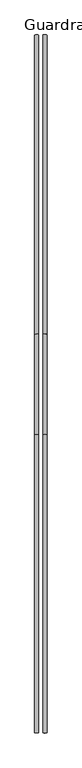
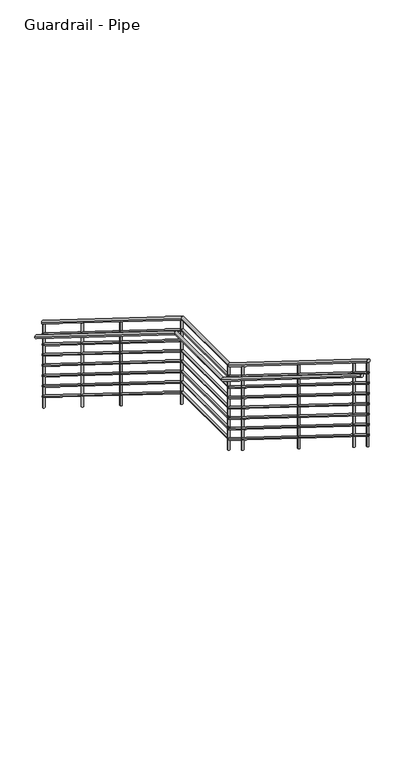
"""IFC4 building model written with IfcOpenShell, lengths in millimetres: railing geometry, Guardrail - Pipe."""

from ifc_helpers import new_model, si_unit, point, frame, frame_2d, origin, place, context, project, spatial, circle_curve, ellipse_curve, trimmed, segment, composite_curve, outline, extrude, source, transform, mapped, element, save
from ifc_brep_helpers import plane_surface, cylinder_surface, advanced_brep


def guardrail_pipe_c5471f49(model_context):
    return source(origin(), model_context, "Body", "SolidModel", [
        advanced_brep(
        [(-2187.3939612, 2884.909643, -2439.0768639), (-2225.4939612, 2884.909643, -2439.0768639), (-2187.3939612, 85.4582154, -693.9642857), (-2225.4939612, 85.4582154, -693.9642857), (-2187.3939612, -854.3417846, -693.9642857), (-2225.4939612, -854.3417846, -693.9642857), (-2187.3939612, -3642.890357, 1044.3517075), (-2225.4939612, -3642.890357, 1044.3517075)],
        [
            (0, 1, ellipse_curve(frame((-2206.4439612, 2884.909643, -2439.0768639), z_axis=(0.0, 1.0, 0.0), x_axis=(0.0, 0.0, -1.0)), 22.4482925, 19.05)),
            (1, 0, ellipse_curve(frame((-2206.4439612, 2884.909643, -2439.0768639), z_axis=(0.0, 1.0, 0.0), x_axis=(0.0, 0.0, -1.0)), 22.4482925, 19.05)),
            (0, 2),
            (2, 3, ellipse_curve(frame((-2206.4439612, 85.4582154, -693.9642857), z_axis=(0.0, 0.9614096116045893, -0.2751209892289441), x_axis=(0.0, -0.27512098922894396, -0.9614096116045893)), 19.8146552, 19.05)),
            (3, 1),
            (3, 2, ellipse_curve(frame((-2206.4439612, 85.4582154, -693.9642857), z_axis=(0.0, 0.9614096116045893, -0.2751209892289441), x_axis=(0.0, -0.27512098922894396, -0.9614096116045893)), 19.8146552, 19.05)),
            (2, 4),
            (4, 5, ellipse_curve(frame((-2206.4439612, -854.3417846, -693.9642857), z_axis=(0.0, 0.9614096116045892, -0.27512098922894423), x_axis=(0.0, 0.2751209892289447, 0.9614096116045893)), 19.8146552, 19.05)),
            (5, 3),
            (5, 4, ellipse_curve(frame((-2206.4439612, -854.3417846, -693.9642857), z_axis=(0.0, 0.9614096116045892, -0.27512098922894423), x_axis=(0.0, 0.2751209892289447, 0.9614096116045893)), 19.8146552, 19.05)),
            (6, 7, ellipse_curve(frame((-2206.4439612, -3642.890357, 1044.3517075), z_axis=(0.0, -1.0, 0.0), x_axis=(0.0, 0.0, -1.0)), 22.4482925, 19.05)),
            (7, 6, ellipse_curve(frame((-2206.4439612, -3642.890357, 1044.3517075), z_axis=(0.0, -1.0, 0.0), x_axis=(0.0, 0.0, -1.0)), 22.4482925, 19.05)),
            (4, 6),
            (7, 5),
        ],
        [
            plane_surface(frame((-2206.4439612, 2884.909643, -2416.6285714), z_axis=(0.0, 1.0, 0.0), x_axis=(0.0, 0.0, -1.0))),
            cylinder_surface(frame((-2206.4439612, 2874.832042, -2432.794723), z_axis=(0.0, 0.8486168825713745, -0.5290079267977392), x_axis=(-1.0, 0.0, 0.0)), 19.05),
            cylinder_surface(frame((-2206.4439612, 90.909643, -693.9642857), z_axis=(0.0, 1.0, 0.0), x_axis=(-1.0, 0.0, 0.0)), 19.05),
            plane_surface(frame((-2206.4439612, -3642.890357, 1066.8), z_axis=(0.0, -1.0, 0.0), x_axis=(0.0, 0.0, -1.0))),
            cylinder_surface(frame((-2206.4439612, -858.967958, -691.0804373), z_axis=(0.0, 0.8486168825713742, -0.5290079267977394), x_axis=(-1.0, 0.0, 0.0)), 19.05),
        ],
        [
            (0, [[1, 2]]),
            (1, [[-1, 3, 4, 5]]),
            (1, [[-2, -5, 6, -3]]),
            (2, [[-4, 7, 8, 9]]),
            (2, [[-6, -9, 10, -7]]),
            (3, [[11, 12]]),
            (4, [[-8, 13, -12, 14]]),
            (4, [[-10, -14, -11, -13]]),
        ],
    ),
        advanced_brep(
        [(-2193.7439612, 2884.909643, -2583.9940998), (-2219.1439612, 2884.909643, -2583.9940998), (-2193.7439612, 87.2753579, -840.0142857), (-2219.1439612, 87.2753579, -840.0142857), (-2193.7439612, -852.5246421, -840.0142857), (-2219.1439612, -852.5246421, -840.0142857), (-2193.7439612, -3642.890357, 899.4344717), (-2219.1439612, -3642.890357, 899.4344717)],
        [
            (0, 1, ellipse_curve(frame((-2206.4439612, 2884.909643, -2583.9940998), z_axis=(0.0, 1.0, 0.0), x_axis=(0.0, 0.0, -1.0)), 14.9655283, 12.7)),
            (1, 0, ellipse_curve(frame((-2206.4439612, 2884.909643, -2583.9940998), z_axis=(0.0, 1.0, 0.0), x_axis=(0.0, 0.0, -1.0)), 14.9655283, 12.7)),
            (0, 2),
            (2, 3, ellipse_curve(frame((-2206.4439612, 87.2753579, -840.0142857), z_axis=(0.0, 0.9614096116045893, -0.2751209892289441), x_axis=(0.0, -0.27512098922894396, -0.9614096116045893)), 13.2097702, 12.7)),
            (3, 1),
            (3, 2, ellipse_curve(frame((-2206.4439612, 87.2753579, -840.0142857), z_axis=(0.0, 0.9614096116045893, -0.2751209892289441), x_axis=(0.0, -0.27512098922894396, -0.9614096116045893)), 13.2097702, 12.7)),
            (2, 4),
            (4, 5, ellipse_curve(frame((-2206.4439612, -852.5246421, -840.0142857), z_axis=(0.0, 0.9614096116045892, -0.27512098922894423), x_axis=(0.0, 0.2751209892289447, 0.9614096116045893)), 13.2097702, 12.7)),
            (5, 3),
            (5, 4, ellipse_curve(frame((-2206.4439612, -852.5246421, -840.0142857), z_axis=(0.0, 0.9614096116045892, -0.27512098922894423), x_axis=(0.0, 0.2751209892289447, 0.9614096116045893)), 13.2097702, 12.7)),
            (6, 7, ellipse_curve(frame((-2206.4439612, -3642.890357, 899.4344717), z_axis=(0.0, -1.0, 0.0), x_axis=(0.0, 0.0, -1.0)), 14.9655283, 12.7)),
            (7, 6, ellipse_curve(frame((-2206.4439612, -3642.890357, 899.4344717), z_axis=(0.0, -1.0, 0.0), x_axis=(0.0, 0.0, -1.0)), 14.9655283, 12.7)),
            (4, 6),
            (7, 5),
        ],
        [
            plane_surface(frame((-2206.4439612, 2884.909643, -2569.0285714), z_axis=(0.0, 1.0, 0.0), x_axis=(0.0, 0.0, -1.0))),
            cylinder_surface(frame((-2206.4439612, 2878.1912423, -2579.8060058), z_axis=(0.0, 0.8486168825713745, -0.5290079267977392), x_axis=(-1.0, 0.0, 0.0)), 12.7),
            cylinder_surface(frame((-2206.4439612, 90.909643, -840.0142857), z_axis=(0.0, 1.0, 0.0), x_axis=(-1.0, 0.0, 0.0)), 12.7),
            plane_surface(frame((-2206.4439612, -3642.890357, 914.4), z_axis=(0.0, -1.0, 0.0), x_axis=(0.0, 0.0, -1.0))),
            cylinder_surface(frame((-2206.4439612, -855.6087577, -838.0917201), z_axis=(0.0, 0.8486168825713742, -0.5290079267977394), x_axis=(-1.0, 0.0, 0.0)), 12.7),
        ],
        [
            (0, [[1, 2]]),
            (1, [[-1, 3, 4, 5]]),
            (1, [[-2, -5, 6, -3]]),
            (2, [[-4, 7, 8, 9]]),
            (2, [[-6, -9, 10, -7]]),
            (3, [[11, 12]]),
            (4, [[-8, 13, -12, 14]]),
            (4, [[-10, -14, -11, -13]]),
        ],
    ),
        advanced_brep(
        [(-2263.5939612, 2884.909643, -2591.4768639), (-2301.6939612, 2884.909643, -2591.4768639), (-2263.5939612, 85.4582154, -846.3642857), (-2301.6939612, 85.4582154, -846.3642857), (-2263.5939612, -854.3417846, -846.3642857), (-2301.6939612, -854.3417846, -846.3642857), (-2263.5939612, -3642.890357, 891.9517075), (-2301.6939612, -3642.890357, 891.9517075)],
        [
            (0, 1, ellipse_curve(frame((-2282.6439612, 2884.909643, -2591.4768639), z_axis=(0.0, 1.0, 0.0), x_axis=(0.0, 0.0, -1.0)), 22.4482925, 19.05)),
            (1, 0, ellipse_curve(frame((-2282.6439612, 2884.909643, -2591.4768639), z_axis=(0.0, 1.0, 0.0), x_axis=(0.0, 0.0, -1.0)), 22.4482925, 19.05)),
            (0, 2),
            (2, 3, ellipse_curve(frame((-2282.6439612, 85.4582154, -846.3642857), z_axis=(0.0, 0.9614096116045893, -0.2751209892289441), x_axis=(0.0, -0.27512098922894396, -0.9614096116045893)), 19.8146552, 19.05)),
            (3, 1),
            (3, 2, ellipse_curve(frame((-2282.6439612, 85.4582154, -846.3642857), z_axis=(0.0, 0.9614096116045893, -0.2751209892289441), x_axis=(0.0, -0.27512098922894396, -0.9614096116045893)), 19.8146552, 19.05)),
            (2, 4),
            (4, 5, ellipse_curve(frame((-2282.6439612, -854.3417846, -846.3642857), z_axis=(0.0, 0.9614096116045892, -0.27512098922894423), x_axis=(0.0, 0.2751209892289447, 0.9614096116045893)), 19.8146552, 19.05)),
            (5, 3),
            (5, 4, ellipse_curve(frame((-2282.6439612, -854.3417846, -846.3642857), z_axis=(0.0, 0.9614096116045892, -0.27512098922894423), x_axis=(0.0, 0.2751209892289447, 0.9614096116045893)), 19.8146552, 19.05)),
            (6, 7, ellipse_curve(frame((-2282.6439612, -3642.890357, 891.9517075), z_axis=(0.0, -1.0, 0.0), x_axis=(0.0, 0.0, -1.0)), 22.4482925, 19.05)),
            (7, 6, ellipse_curve(frame((-2282.6439612, -3642.890357, 891.9517075), z_axis=(0.0, -1.0, 0.0), x_axis=(0.0, 0.0, -1.0)), 22.4482925, 19.05)),
            (4, 6),
            (7, 5),
        ],
        [
            plane_surface(frame((-2282.6439612, 2884.909643, -2569.0285714), z_axis=(0.0, 1.0, 0.0), x_axis=(0.0, 0.0, -1.0))),
            cylinder_surface(frame((-2282.6439612, 2874.832042, -2585.194723), z_axis=(0.0, 0.8486168825713745, -0.5290079267977392), x_axis=(-1.0, 0.0, 0.0)), 19.05),
            cylinder_surface(frame((-2282.6439612, 90.909643, -846.3642857), z_axis=(0.0, 1.0, 0.0), x_axis=(-1.0, 0.0, 0.0)), 19.05),
            plane_surface(frame((-2282.6439612, -3642.890357, 914.4), z_axis=(0.0, -1.0, 0.0), x_axis=(0.0, 0.0, -1.0))),
            cylinder_surface(frame((-2282.6439612, -858.967958, -843.4804373), z_axis=(0.0, 0.8486168825713742, -0.5290079267977394), x_axis=(-1.0, 0.0, 0.0)), 19.05),
        ],
        [
            (0, [[1, 2]]),
            (1, [[-1, 3, 4, 5]]),
            (1, [[-2, -5, 6, -3]]),
            (2, [[-4, 7, 8, 9]]),
            (2, [[-6, -9, 10, -7]]),
            (3, [[11, 12]]),
            (4, [[-8, 13, -12, 14]]),
            (4, [[-10, -14, -11, -13]]),
        ],
    ),
        advanced_brep(
        [(-2193.7439612, 2884.909643, -2710.9940998), (-2219.1439612, 2884.909643, -2710.9940998), (-2193.7439612, 87.2753579, -967.0142857), (-2219.1439612, 87.2753579, -967.0142857), (-2193.7439612, -852.5246421, -967.0142857), (-2219.1439612, -852.5246421, -967.0142857), (-2193.7439612, -3642.890357, 772.4344717), (-2219.1439612, -3642.890357, 772.4344717)],
        [
            (0, 1, ellipse_curve(frame((-2206.4439612, 2884.909643, -2710.9940998), z_axis=(0.0, 1.0, 0.0), x_axis=(0.0, 0.0, -1.0)), 14.9655283, 12.7)),
            (1, 0, ellipse_curve(frame((-2206.4439612, 2884.909643, -2710.9940998), z_axis=(0.0, 1.0, 0.0), x_axis=(0.0, 0.0, -1.0)), 14.9655283, 12.7)),
            (0, 2),
            (2, 3, ellipse_curve(frame((-2206.4439612, 87.2753579, -967.0142857), z_axis=(0.0, 0.9614096116045893, -0.2751209892289441), x_axis=(0.0, -0.27512098922894396, -0.9614096116045893)), 13.2097702, 12.7)),
            (3, 1),
            (3, 2, ellipse_curve(frame((-2206.4439612, 87.2753579, -967.0142857), z_axis=(0.0, 0.9614096116045893, -0.2751209892289441), x_axis=(0.0, -0.27512098922894396, -0.9614096116045893)), 13.2097702, 12.7)),
            (2, 4),
            (4, 5, ellipse_curve(frame((-2206.4439612, -852.5246421, -967.0142857), z_axis=(0.0, 0.9614096116045892, -0.27512098922894423), x_axis=(0.0, 0.2751209892289447, 0.9614096116045893)), 13.2097702, 12.7)),
            (5, 3),
            (5, 4, ellipse_curve(frame((-2206.4439612, -852.5246421, -967.0142857), z_axis=(0.0, 0.9614096116045892, -0.27512098922894423), x_axis=(0.0, 0.2751209892289447, 0.9614096116045893)), 13.2097702, 12.7)),
            (6, 7, ellipse_curve(frame((-2206.4439612, -3642.890357, 772.4344717), z_axis=(0.0, -1.0, 0.0), x_axis=(0.0, 0.0, -1.0)), 14.9655283, 12.7)),
            (7, 6, ellipse_curve(frame((-2206.4439612, -3642.890357, 772.4344717), z_axis=(0.0, -1.0, 0.0), x_axis=(0.0, 0.0, -1.0)), 14.9655283, 12.7)),
            (4, 6),
            (7, 5),
        ],
        [
            plane_surface(frame((-2206.4439612, 2884.909643, -2696.0285714), z_axis=(0.0, 1.0, 0.0), x_axis=(0.0, 0.0, -1.0))),
            cylinder_surface(frame((-2206.4439612, 2878.1912423, -2706.8060058), z_axis=(0.0, 0.8486168825713745, -0.5290079267977392), x_axis=(-1.0, 0.0, 0.0)), 12.7),
            cylinder_surface(frame((-2206.4439612, 90.909643, -967.0142857), z_axis=(0.0, 1.0, 0.0), x_axis=(-1.0, 0.0, 0.0)), 12.7),
            plane_surface(frame((-2206.4439612, -3642.890357, 787.4), z_axis=(0.0, -1.0, 0.0), x_axis=(0.0, 0.0, -1.0))),
            cylinder_surface(frame((-2206.4439612, -855.6087577, -965.0917201), z_axis=(0.0, 0.8486168825713742, -0.5290079267977394), x_axis=(-1.0, 0.0, 0.0)), 12.7),
        ],
        [
            (0, [[1, 2]]),
            (1, [[-1, 3, 4, 5]]),
            (1, [[-2, -5, 6, -3]]),
            (2, [[-4, 7, 8, 9]]),
            (2, [[-6, -9, 10, -7]]),
            (3, [[11, 12]]),
            (4, [[-8, 13, -12, 14]]),
            (4, [[-10, -14, -11, -13]]),
        ],
    ),
        advanced_brep(
        [(-2193.7439612, 2884.909643, -2837.9940998), (-2219.1439612, 2884.909643, -2837.9940998), (-2193.7439612, 87.2753579, -1094.0142857), (-2219.1439612, 87.2753579, -1094.0142857), (-2193.7439612, -852.5246421, -1094.0142857), (-2219.1439612, -852.5246421, -1094.0142857), (-2193.7439612, -3642.890357, 645.4344717), (-2219.1439612, -3642.890357, 645.4344717)],
        [
            (0, 1, ellipse_curve(frame((-2206.4439612, 2884.909643, -2837.9940998), z_axis=(0.0, 1.0, 0.0), x_axis=(0.0, 0.0, -1.0)), 14.9655283, 12.7)),
            (1, 0, ellipse_curve(frame((-2206.4439612, 2884.909643, -2837.9940998), z_axis=(0.0, 1.0, 0.0), x_axis=(0.0, 0.0, -1.0)), 14.9655283, 12.7)),
            (0, 2),
            (2, 3, ellipse_curve(frame((-2206.4439612, 87.2753579, -1094.0142857), z_axis=(0.0, 0.9614096116045893, -0.2751209892289441), x_axis=(0.0, -0.27512098922894396, -0.9614096116045893)), 13.2097702, 12.7)),
            (3, 1),
            (3, 2, ellipse_curve(frame((-2206.4439612, 87.2753579, -1094.0142857), z_axis=(0.0, 0.9614096116045893, -0.2751209892289441), x_axis=(0.0, -0.27512098922894396, -0.9614096116045893)), 13.2097702, 12.7)),
            (2, 4),
            (4, 5, ellipse_curve(frame((-2206.4439612, -852.5246421, -1094.0142857), z_axis=(0.0, 0.9614096116045892, -0.27512098922894423), x_axis=(0.0, 0.2751209892289447, 0.9614096116045893)), 13.2097702, 12.7)),
            (5, 3),
            (5, 4, ellipse_curve(frame((-2206.4439612, -852.5246421, -1094.0142857), z_axis=(0.0, 0.9614096116045892, -0.27512098922894423), x_axis=(0.0, 0.2751209892289447, 0.9614096116045893)), 13.2097702, 12.7)),
            (6, 7, ellipse_curve(frame((-2206.4439612, -3642.890357, 645.4344717), z_axis=(0.0, -1.0, 0.0), x_axis=(0.0, 0.0, -1.0)), 14.9655283, 12.7)),
            (7, 6, ellipse_curve(frame((-2206.4439612, -3642.890357, 645.4344717), z_axis=(0.0, -1.0, 0.0), x_axis=(0.0, 0.0, -1.0)), 14.9655283, 12.7)),
            (4, 6),
            (7, 5),
        ],
        [
            plane_surface(frame((-2206.4439612, 2884.909643, -2823.0285714), z_axis=(0.0, 1.0, 0.0), x_axis=(0.0, 0.0, -1.0))),
            cylinder_surface(frame((-2206.4439612, 2878.1912423, -2833.8060058), z_axis=(0.0, 0.8486168825713745, -0.5290079267977392), x_axis=(-1.0, 0.0, 0.0)), 12.7),
            cylinder_surface(frame((-2206.4439612, 90.909643, -1094.0142857), z_axis=(0.0, 1.0, 0.0), x_axis=(-1.0, 0.0, 0.0)), 12.7),
            plane_surface(frame((-2206.4439612, -3642.890357, 660.4), z_axis=(0.0, -1.0, 0.0), x_axis=(0.0, 0.0, -1.0))),
            cylinder_surface(frame((-2206.4439612, -855.6087577, -1092.0917201), z_axis=(0.0, 0.8486168825713742, -0.5290079267977394), x_axis=(-1.0, 0.0, 0.0)), 12.7),
        ],
        [
            (0, [[1, 2]]),
            (1, [[-1, 3, 4, 5]]),
            (1, [[-2, -5, 6, -3]]),
            (2, [[-4, 7, 8, 9]]),
            (2, [[-6, -9, 10, -7]]),
            (3, [[11, 12]]),
            (4, [[-8, 13, -12, 14]]),
            (4, [[-10, -14, -11, -13]]),
        ],
    ),
        advanced_brep(
        [(-2193.7439612, 2884.909643, -2964.9940998), (-2219.1439612, 2884.909643, -2964.9940998), (-2193.7439612, 87.2753579, -1221.0142857), (-2219.1439612, 87.2753579, -1221.0142857), (-2193.7439612, -852.5246421, -1221.0142857), (-2219.1439612, -852.5246421, -1221.0142857), (-2193.7439612, -3642.890357, 518.4344717), (-2219.1439612, -3642.890357, 518.4344717)],
        [
            (0, 1, ellipse_curve(frame((-2206.4439612, 2884.909643, -2964.9940998), z_axis=(0.0, 1.0, 0.0), x_axis=(0.0, 0.0, -1.0)), 14.9655283, 12.7)),
            (1, 0, ellipse_curve(frame((-2206.4439612, 2884.909643, -2964.9940998), z_axis=(0.0, 1.0, 0.0), x_axis=(0.0, 0.0, -1.0)), 14.9655283, 12.7)),
            (0, 2),
            (2, 3, ellipse_curve(frame((-2206.4439612, 87.2753579, -1221.0142857), z_axis=(0.0, 0.9614096116045893, -0.2751209892289441), x_axis=(0.0, -0.27512098922894396, -0.9614096116045893)), 13.2097702, 12.7)),
            (3, 1),
            (3, 2, ellipse_curve(frame((-2206.4439612, 87.2753579, -1221.0142857), z_axis=(0.0, 0.9614096116045893, -0.2751209892289441), x_axis=(0.0, -0.27512098922894396, -0.9614096116045893)), 13.2097702, 12.7)),
            (2, 4),
            (4, 5, ellipse_curve(frame((-2206.4439612, -852.5246421, -1221.0142857), z_axis=(0.0, 0.9614096116045892, -0.27512098922894423), x_axis=(0.0, 0.2751209892289447, 0.9614096116045893)), 13.2097702, 12.7)),
            (5, 3),
            (5, 4, ellipse_curve(frame((-2206.4439612, -852.5246421, -1221.0142857), z_axis=(0.0, 0.9614096116045892, -0.27512098922894423), x_axis=(0.0, 0.2751209892289447, 0.9614096116045893)), 13.2097702, 12.7)),
            (6, 7, ellipse_curve(frame((-2206.4439612, -3642.890357, 518.4344717), z_axis=(0.0, -1.0, 0.0), x_axis=(0.0, 0.0, -1.0)), 14.9655283, 12.7)),
            (7, 6, ellipse_curve(frame((-2206.4439612, -3642.890357, 518.4344717), z_axis=(0.0, -1.0, 0.0), x_axis=(0.0, 0.0, -1.0)), 14.9655283, 12.7)),
            (4, 6),
            (7, 5),
        ],
        [
            plane_surface(frame((-2206.4439612, 2884.909643, -2950.0285714), z_axis=(0.0, 1.0, 0.0), x_axis=(0.0, 0.0, -1.0))),
            cylinder_surface(frame((-2206.4439612, 2878.1912423, -2960.8060058), z_axis=(0.0, 0.8486168825713745, -0.5290079267977392), x_axis=(-1.0, 0.0, 0.0)), 12.7),
            cylinder_surface(frame((-2206.4439612, 90.909643, -1221.0142857), z_axis=(0.0, 1.0, 0.0), x_axis=(-1.0, 0.0, 0.0)), 12.7),
            plane_surface(frame((-2206.4439612, -3642.890357, 533.4), z_axis=(0.0, -1.0, 0.0), x_axis=(0.0, 0.0, -1.0))),
            cylinder_surface(frame((-2206.4439612, -855.6087577, -1219.0917201), z_axis=(0.0, 0.8486168825713742, -0.5290079267977394), x_axis=(-1.0, 0.0, 0.0)), 12.7),
        ],
        [
            (0, [[1, 2]]),
            (1, [[-1, 3, 4, 5]]),
            (1, [[-2, -5, 6, -3]]),
            (2, [[-4, 7, 8, 9]]),
            (2, [[-6, -9, 10, -7]]),
            (3, [[11, 12]]),
            (4, [[-8, 13, -12, 14]]),
            (4, [[-10, -14, -11, -13]]),
        ],
    ),
        advanced_brep(
        [(-2193.7439612, 2884.909643, -3091.9940998), (-2219.1439612, 2884.909643, -3091.9940998), (-2193.7439612, 87.2753579, -1348.0142857), (-2219.1439612, 87.2753579, -1348.0142857), (-2193.7439612, -852.5246421, -1348.0142857), (-2219.1439612, -852.5246421, -1348.0142857), (-2193.7439612, -3642.890357, 391.4344717), (-2219.1439612, -3642.890357, 391.4344717)],
        [
            (0, 1, ellipse_curve(frame((-2206.4439612, 2884.909643, -3091.9940998), z_axis=(0.0, 1.0, 0.0), x_axis=(0.0, 0.0, -1.0)), 14.9655283, 12.7)),
            (1, 0, ellipse_curve(frame((-2206.4439612, 2884.909643, -3091.9940998), z_axis=(0.0, 1.0, 0.0), x_axis=(0.0, 0.0, -1.0)), 14.9655283, 12.7)),
            (0, 2),
            (2, 3, ellipse_curve(frame((-2206.4439612, 87.2753579, -1348.0142857), z_axis=(0.0, 0.9614096116045893, -0.2751209892289441), x_axis=(0.0, -0.27512098922894396, -0.9614096116045893)), 13.2097702, 12.7)),
            (3, 1),
            (3, 2, ellipse_curve(frame((-2206.4439612, 87.2753579, -1348.0142857), z_axis=(0.0, 0.9614096116045893, -0.2751209892289441), x_axis=(0.0, -0.27512098922894396, -0.9614096116045893)), 13.2097702, 12.7)),
            (2, 4),
            (4, 5, ellipse_curve(frame((-2206.4439612, -852.5246421, -1348.0142857), z_axis=(0.0, 0.9614096116045892, -0.27512098922894423), x_axis=(0.0, 0.2751209892289447, 0.9614096116045893)), 13.2097702, 12.7)),
            (5, 3),
            (5, 4, ellipse_curve(frame((-2206.4439612, -852.5246421, -1348.0142857), z_axis=(0.0, 0.9614096116045892, -0.27512098922894423), x_axis=(0.0, 0.2751209892289447, 0.9614096116045893)), 13.2097702, 12.7)),
            (6, 7, ellipse_curve(frame((-2206.4439612, -3642.890357, 391.4344717), z_axis=(0.0, -1.0, 0.0), x_axis=(0.0, 0.0, -1.0)), 14.9655283, 12.7)),
            (7, 6, ellipse_curve(frame((-2206.4439612, -3642.890357, 391.4344717), z_axis=(0.0, -1.0, 0.0), x_axis=(0.0, 0.0, -1.0)), 14.9655283, 12.7)),
            (4, 6),
            (7, 5),
        ],
        [
            plane_surface(frame((-2206.4439612, 2884.909643, -3077.0285714), z_axis=(0.0, 1.0, 0.0), x_axis=(0.0, 0.0, -1.0))),
            cylinder_surface(frame((-2206.4439612, 2878.1912423, -3087.8060058), z_axis=(0.0, 0.8486168825713745, -0.5290079267977392), x_axis=(-1.0, 0.0, 0.0)), 12.7),
            cylinder_surface(frame((-2206.4439612, 90.909643, -1348.0142857), z_axis=(0.0, 1.0, 0.0), x_axis=(-1.0, 0.0, 0.0)), 12.7),
            plane_surface(frame((-2206.4439612, -3642.890357, 406.4), z_axis=(0.0, -1.0, 0.0), x_axis=(0.0, 0.0, -1.0))),
            cylinder_surface(frame((-2206.4439612, -855.6087577, -1346.0917201), z_axis=(0.0, 0.8486168825713742, -0.5290079267977394), x_axis=(-1.0, 0.0, 0.0)), 12.7),
        ],
        [
            (0, [[1, 2]]),
            (1, [[-1, 3, 4, 5]]),
            (1, [[-2, -5, 6, -3]]),
            (2, [[-4, 7, 8, 9]]),
            (2, [[-6, -9, 10, -7]]),
            (3, [[11, 12]]),
            (4, [[-8, 13, -12, 14]]),
            (4, [[-10, -14, -11, -13]]),
        ],
    ),
        advanced_brep(
        [(-2193.7439612, 2884.909643, -3218.9940998), (-2219.1439612, 2884.909643, -3218.9940998), (-2193.7439612, 87.2753579, -1475.0142857), (-2219.1439612, 87.2753579, -1475.0142857), (-2193.7439612, -852.5246421, -1475.0142857), (-2219.1439612, -852.5246421, -1475.0142857), (-2193.7439612, -3642.890357, 264.4344717), (-2219.1439612, -3642.890357, 264.4344717)],
        [
            (0, 1, ellipse_curve(frame((-2206.4439612, 2884.909643, -3218.9940998), z_axis=(0.0, 1.0, 0.0), x_axis=(0.0, 0.0, -1.0)), 14.9655283, 12.7)),
            (1, 0, ellipse_curve(frame((-2206.4439612, 2884.909643, -3218.9940998), z_axis=(0.0, 1.0, 0.0), x_axis=(0.0, 0.0, -1.0)), 14.9655283, 12.7)),
            (0, 2),
            (2, 3, ellipse_curve(frame((-2206.4439612, 87.2753579, -1475.0142857), z_axis=(0.0, 0.9614096116045893, -0.2751209892289441), x_axis=(0.0, -0.27512098922894396, -0.9614096116045893)), 13.2097702, 12.7)),
            (3, 1),
            (3, 2, ellipse_curve(frame((-2206.4439612, 87.2753579, -1475.0142857), z_axis=(0.0, 0.9614096116045893, -0.2751209892289441), x_axis=(0.0, -0.27512098922894396, -0.9614096116045893)), 13.2097702, 12.7)),
            (2, 4),
            (4, 5, ellipse_curve(frame((-2206.4439612, -852.5246421, -1475.0142857), z_axis=(0.0, 0.9614096116045892, -0.27512098922894423), x_axis=(0.0, 0.2751209892289447, 0.9614096116045893)), 13.2097702, 12.7)),
            (5, 3),
            (5, 4, ellipse_curve(frame((-2206.4439612, -852.5246421, -1475.0142857), z_axis=(0.0, 0.9614096116045892, -0.27512098922894423), x_axis=(0.0, 0.2751209892289447, 0.9614096116045893)), 13.2097702, 12.7)),
            (6, 7, ellipse_curve(frame((-2206.4439612, -3642.890357, 264.4344717), z_axis=(0.0, -1.0, 0.0), x_axis=(0.0, 0.0, -1.0)), 14.9655283, 12.7)),
            (7, 6, ellipse_curve(frame((-2206.4439612, -3642.890357, 264.4344717), z_axis=(0.0, -1.0, 0.0), x_axis=(0.0, 0.0, -1.0)), 14.9655283, 12.7)),
            (4, 6),
            (7, 5),
        ],
        [
            plane_surface(frame((-2206.4439612, 2884.909643, -3204.0285714), z_axis=(0.0, 1.0, 0.0), x_axis=(0.0, 0.0, -1.0))),
            cylinder_surface(frame((-2206.4439612, 2878.1912423, -3214.8060058), z_axis=(0.0, 0.8486168825713745, -0.5290079267977392), x_axis=(-1.0, 0.0, 0.0)), 12.7),
            cylinder_surface(frame((-2206.4439612, 90.909643, -1475.0142857), z_axis=(0.0, 1.0, 0.0), x_axis=(-1.0, 0.0, 0.0)), 12.7),
            plane_surface(frame((-2206.4439612, -3642.890357, 279.4), z_axis=(0.0, -1.0, 0.0), x_axis=(0.0, 0.0, -1.0))),
            cylinder_surface(frame((-2206.4439612, -855.6087577, -1473.0917201), z_axis=(0.0, 0.8486168825713742, -0.5290079267977394), x_axis=(-1.0, 0.0, 0.0)), 12.7),
        ],
        [
            (0, [[1, 2]]),
            (1, [[-1, 3, 4, 5]]),
            (1, [[-2, -5, 6, -3]]),
            (2, [[-4, 7, 8, 9]]),
            (2, [[-6, -9, 10, -7]]),
            (3, [[11, 12]]),
            (4, [[-8, 13, -12, 14]]),
            (4, [[-10, -14, -11, -13]]),
        ],
    ),
        advanced_brep(
        [(-2193.7439612, 2884.909643, -3345.9940998), (-2219.1439612, 2884.909643, -3345.9940998), (-2193.7439612, 87.2753579, -1602.0142857), (-2219.1439612, 87.2753579, -1602.0142857), (-2193.7439612, -852.5246421, -1602.0142857), (-2219.1439612, -852.5246421, -1602.0142857), (-2193.7439612, -3642.890357, 137.4344717), (-2219.1439612, -3642.890357, 137.4344717)],
        [
            (0, 1, ellipse_curve(frame((-2206.4439612, 2884.909643, -3345.9940998), z_axis=(0.0, 1.0, 0.0), x_axis=(0.0, 0.0, -1.0)), 14.9655283, 12.7)),
            (1, 0, ellipse_curve(frame((-2206.4439612, 2884.909643, -3345.9940998), z_axis=(0.0, 1.0, 0.0), x_axis=(0.0, 0.0, -1.0)), 14.9655283, 12.7)),
            (0, 2),
            (2, 3, ellipse_curve(frame((-2206.4439612, 87.2753579, -1602.0142857), z_axis=(0.0, 0.9614096116045893, -0.2751209892289441), x_axis=(0.0, -0.27512098922894396, -0.9614096116045893)), 13.2097702, 12.7)),
            (3, 1),
            (3, 2, ellipse_curve(frame((-2206.4439612, 87.2753579, -1602.0142857), z_axis=(0.0, 0.9614096116045893, -0.2751209892289441), x_axis=(0.0, -0.27512098922894396, -0.9614096116045893)), 13.2097702, 12.7)),
            (2, 4),
            (4, 5, ellipse_curve(frame((-2206.4439612, -852.5246421, -1602.0142857), z_axis=(0.0, 0.9614096116045892, -0.27512098922894423), x_axis=(0.0, 0.2751209892289447, 0.9614096116045893)), 13.2097702, 12.7)),
            (5, 3),
            (5, 4, ellipse_curve(frame((-2206.4439612, -852.5246421, -1602.0142857), z_axis=(0.0, 0.9614096116045892, -0.27512098922894423), x_axis=(0.0, 0.2751209892289447, 0.9614096116045893)), 13.2097702, 12.7)),
            (6, 7, ellipse_curve(frame((-2206.4439612, -3642.890357, 137.4344717), z_axis=(0.0, -1.0, 0.0), x_axis=(0.0, 0.0, -1.0)), 14.9655283, 12.7)),
            (7, 6, ellipse_curve(frame((-2206.4439612, -3642.890357, 137.4344717), z_axis=(0.0, -1.0, 0.0), x_axis=(0.0, 0.0, -1.0)), 14.9655283, 12.7)),
            (4, 6),
            (7, 5),
        ],
        [
            plane_surface(frame((-2206.4439612, 2884.909643, -3331.0285714), z_axis=(0.0, 1.0, 0.0), x_axis=(0.0, 0.0, -1.0))),
            cylinder_surface(frame((-2206.4439612, 2878.1912423, -3341.8060058), z_axis=(0.0, 0.8486168825713745, -0.5290079267977392), x_axis=(-1.0, 0.0, 0.0)), 12.7),
            cylinder_surface(frame((-2206.4439612, 90.909643, -1602.0142857), z_axis=(0.0, 1.0, 0.0), x_axis=(-1.0, 0.0, 0.0)), 12.7),
            plane_surface(frame((-2206.4439612, -3642.890357, 152.4), z_axis=(0.0, -1.0, 0.0), x_axis=(0.0, 0.0, -1.0))),
            cylinder_surface(frame((-2206.4439612, -855.6087577, -1600.0917201), z_axis=(0.0, 0.8486168825713742, -0.5290079267977394), x_axis=(-1.0, 0.0, 0.0)), 12.7),
        ],
        [
            (0, [[1, 2]]),
            (1, [[-1, 3, 4, 5]]),
            (1, [[-2, -5, 6, -3]]),
            (2, [[-4, 7, 8, 9]]),
            (2, [[-6, -9, 10, -7]]),
            (3, [[11, 12]]),
            (4, [[-8, 13, -12, 14]]),
            (4, [[-10, -14, -11, -13]]),
        ],
    ),
        advanced_brep(
        [(-2219.1439612, -3630.5087726, -7.7183903), (-2193.7439612, -3630.5087726, -7.7183903), (-2193.7439612, -3630.5087726, 1014.1850247), (-2219.1439612, -3630.5087726, 1014.1850247)],
        [
            (0, 1, circle_curve(frame((-2206.4439612, -3630.5087726, -7.7183903), z_axis=(0.0, 0.0, -1.0), x_axis=(1.0, 0.0, 0.0)), 12.7)),
            (1, 0, circle_curve(frame((-2206.4439612, -3630.5087726, -7.7183903), z_axis=(0.0, 0.0, -1.0), x_axis=(1.0, 0.0, 0.0)), 12.7)),
            (1, 2),
            (2, 3, ellipse_curve(frame((-2206.4439612, -3630.5087726, 1014.1850247), z_axis=(0.0, -0.5290079267977408, -0.8486168825713734), x_axis=(0.0, -0.8486168825713732, 0.5290079267977408)), 14.9655283, 12.7)),
            (3, 0),
            (3, 2, ellipse_curve(frame((-2206.4439612, -3630.5087726, 1014.1850247), z_axis=(0.0, -0.5290079267977408, -0.8486168825713734), x_axis=(0.0, -0.8486168825713732, 0.5290079267977408)), 14.9655283, 12.7)),
        ],
        [
            plane_surface(frame((-2193.7439612, -3630.5087726, -7.7183903), z_axis=(0.0, 0.0, -1.0), x_axis=(0.0, -1.0, 0.0))),
            cylinder_surface(frame((-2206.4439612, -3630.5087726, -7.7183903), z_axis=(0.0, 0.0, 1.0), x_axis=(1.0, 0.0, 0.0)), 12.7),
            plane_surface(frame((-2159.2181313, -3665.4337726, 1035.9564532), z_axis=(0.0, 0.5290079267977408, 0.8486168825713734), x_axis=(-1.0, 0.0, 0.0))),
        ],
        [
            (0, [[1, 2]]),
            (1, [[-2, 3, 4, 5]]),
            (1, [[-1, -5, 6, -3]]),
            (2, [[-4, -6]]),
        ],
    ),
        advanced_brep(
        [(-2219.1439612, -3351.1087726, -181.8898189), (-2193.7439612, -3351.1087726, -181.8898189), (-2193.7439612, -3351.1087726, 840.0135961), (-2219.1439612, -3351.1087726, 840.0135961)],
        [
            (0, 1, circle_curve(frame((-2206.4439612, -3351.1087726, -181.8898189), z_axis=(0.0, 0.0, -1.0), x_axis=(1.0, 0.0, 0.0)), 12.7)),
            (1, 0, circle_curve(frame((-2206.4439612, -3351.1087726, -181.8898189), z_axis=(0.0, 0.0, -1.0), x_axis=(1.0, 0.0, 0.0)), 12.7)),
            (1, 2),
            (2, 3, ellipse_curve(frame((-2206.4439612, -3351.1087726, 840.0135961), z_axis=(0.0, -0.5290079267977408, -0.8486168825713734), x_axis=(0.0, -0.8486168825713732, 0.5290079267977408)), 14.9655283, 12.7)),
            (3, 0),
            (3, 2, ellipse_curve(frame((-2206.4439612, -3351.1087726, 840.0135961), z_axis=(0.0, -0.5290079267977408, -0.8486168825713734), x_axis=(0.0, -0.8486168825713732, 0.5290079267977408)), 14.9655283, 12.7)),
        ],
        [
            plane_surface(frame((-2193.7439612, -3351.1087726, -181.8898189), z_axis=(0.0, 0.0, -1.0), x_axis=(0.0, -1.0, 0.0))),
            cylinder_surface(frame((-2206.4439612, -3351.1087726, -181.8898189), z_axis=(0.0, 0.0, 1.0), x_axis=(1.0, 0.0, 0.0)), 12.7),
            plane_surface(frame((-2159.2181313, -3386.0337726, 861.7850247), z_axis=(0.0, 0.5290079267977408, 0.8486168825713734), x_axis=(-1.0, 0.0, 0.0))),
        ],
        [
            (0, [[1, 2]]),
            (1, [[-2, 3, 4, 5]]),
            (1, [[-1, -5, 6, -3]]),
            (2, [[-4, -6]]),
        ],
    ),
        advanced_brep(
        [(-2219.1439612, -2245.890357, -870.8571429), (-2193.7439612, -2245.890357, -870.8571429), (-2193.7439612, -2245.890357, 151.0462721), (-2219.1439612, -2245.890357, 151.0462721)],
        [
            (0, 1, circle_curve(frame((-2206.4439612, -2245.890357, -870.8571429), z_axis=(0.0, 0.0, -1.0), x_axis=(1.0, 0.0, 0.0)), 12.7)),
            (1, 0, circle_curve(frame((-2206.4439612, -2245.890357, -870.8571429), z_axis=(0.0, 0.0, -1.0), x_axis=(1.0, 0.0, 0.0)), 12.7)),
            (1, 2),
            (2, 3, ellipse_curve(frame((-2206.4439612, -2245.890357, 151.0462721), z_axis=(0.0, -0.5290079267977408, -0.8486168825713734), x_axis=(0.0, -0.8486168825713732, 0.5290079267977408)), 14.9655283, 12.7)),
            (3, 0),
            (3, 2, ellipse_curve(frame((-2206.4439612, -2245.890357, 151.0462721), z_axis=(0.0, -0.5290079267977408, -0.8486168825713734), x_axis=(0.0, -0.8486168825713732, 0.5290079267977408)), 14.9655283, 12.7)),
        ],
        [
            plane_surface(frame((-2193.7439612, -2245.890357, -870.8571429), z_axis=(0.0, 0.0, -1.0), x_axis=(0.0, -1.0, 0.0))),
            cylinder_surface(frame((-2206.4439612, -2245.890357, -870.8571429), z_axis=(0.0, 0.0, 1.0), x_axis=(1.0, 0.0, 0.0)), 12.7),
            plane_surface(frame((-2159.2181313, -2280.815357, 172.8177007), z_axis=(0.0, 0.5290079267977408, 0.8486168825713734), x_axis=(-1.0, 0.0, 0.0))),
        ],
        [
            (0, [[1, 2]]),
            (1, [[-2, 3, 4, 5]]),
            (1, [[-1, -5, 6, -3]]),
            (2, [[-4, -6]]),
        ],
    ),
        advanced_brep(
        [(-2219.1439612, -1115.9087726, -1575.2612475), (-2193.7439612, -1115.9087726, -1575.2612475), (-2193.7439612, -1115.9087726, -553.3578325), (-2219.1439612, -1115.9087726, -553.3578325)],
        [
            (0, 1, circle_curve(frame((-2206.4439612, -1115.9087726, -1575.2612475), z_axis=(0.0, 0.0, -1.0), x_axis=(1.0, 0.0, 0.0)), 12.7)),
            (1, 0, circle_curve(frame((-2206.4439612, -1115.9087726, -1575.2612475), z_axis=(0.0, 0.0, -1.0), x_axis=(1.0, 0.0, 0.0)), 12.7)),
            (1, 2),
            (2, 3, ellipse_curve(frame((-2206.4439612, -1115.9087726, -553.3578325), z_axis=(0.0, -0.5290079267977408, -0.8486168825713734), x_axis=(0.0, -0.8486168825713732, 0.5290079267977408)), 14.9655283, 12.7)),
            (3, 0),
            (3, 2, ellipse_curve(frame((-2206.4439612, -1115.9087726, -553.3578325), z_axis=(0.0, -0.5290079267977408, -0.8486168825713734), x_axis=(0.0, -0.8486168825713732, 0.5290079267977408)), 14.9655283, 12.7)),
        ],
        [
            plane_surface(frame((-2193.7439612, -1115.9087726, -1575.2612475), z_axis=(0.0, 0.0, -1.0), x_axis=(0.0, -1.0, 0.0))),
            cylinder_surface(frame((-2206.4439612, -1115.9087726, -1575.2612475), z_axis=(0.0, 0.0, 1.0), x_axis=(1.0, 0.0, 0.0)), 12.7),
            plane_surface(frame((-2159.2181313, -1150.8337726, -531.5864039), z_axis=(0.0, 0.5290079267977408, 0.8486168825713734), x_axis=(-1.0, 0.0, 0.0))),
        ],
        [
            (0, [[1, 2]]),
            (1, [[-2, 3, 4, 5]]),
            (1, [[-1, -5, 6, -3]]),
            (2, [[-4, -6]]),
        ],
    ),
        extrude(outline(composite_curve([segment(trimmed(circle_curve(frame_2d((-2206.4439612, -836.5087726)), 12.7), [point((-2219.1439612, -836.5087726))], [point((-2193.7439612, -836.5087726))], False, "CARTESIAN"), True, "CONTINUOUS"), segment(trimmed(circle_curve(frame_2d((-2206.4439612, -836.5087726)), 12.7), [point((-2193.7439612, -836.5087726))], [point((-2219.1439612, -836.5087726))], False, "CARTESIAN"), True, "CONTINUOUS")], self_intersect=False)), frame((0.0, 0.0, -1741.7142857), z_axis=(0.0, 0.0, 1.0), x_axis=(1.0, 0.0, 0.0)), (0.0, 0.0, 1.0), 1028.7),
        advanced_brep(
        [(-2219.1439612, 103.2912274, -1749.432676), (-2193.7439612, 103.2912274, -1749.432676), (-2193.7439612, 103.2912274, -727.529261), (-2219.1439612, 103.2912274, -727.529261)],
        [
            (0, 1, circle_curve(frame((-2206.4439612, 103.2912274, -1749.432676), z_axis=(0.0, 0.0, -1.0), x_axis=(1.0, 0.0, 0.0)), 12.7)),
            (1, 0, circle_curve(frame((-2206.4439612, 103.2912274, -1749.432676), z_axis=(0.0, 0.0, -1.0), x_axis=(1.0, 0.0, 0.0)), 12.7)),
            (1, 2),
            (2, 3, ellipse_curve(frame((-2206.4439612, 103.2912274, -727.529261), z_axis=(0.0, -0.5290079267977408, -0.8486168825713734), x_axis=(0.0, -0.8486168825713732, 0.5290079267977408)), 14.9655283, 12.7)),
            (3, 0),
            (3, 2, ellipse_curve(frame((-2206.4439612, 103.2912274, -727.529261), z_axis=(0.0, -0.5290079267977408, -0.8486168825713734), x_axis=(0.0, -0.8486168825713732, 0.5290079267977408)), 14.9655283, 12.7)),
        ],
        [
            plane_surface(frame((-2193.7439612, 103.2912274, -1749.432676), z_axis=(0.0, 0.0, -1.0), x_axis=(0.0, -1.0, 0.0))),
            cylinder_surface(frame((-2206.4439612, 103.2912274, -1749.432676), z_axis=(0.0, 0.0, 1.0), x_axis=(1.0, 0.0, 0.0)), 12.7),
            plane_surface(frame((-2159.2181313, 68.3662274, -705.7578325), z_axis=(0.0, 0.5290079267977408, 0.8486168825713734), x_axis=(-1.0, 0.0, 0.0))),
        ],
        [
            (0, [[1, 2]]),
            (1, [[-2, 3, 4, 5]]),
            (1, [[-1, -5, 6, -3]]),
            (2, [[-4, -6]]),
        ],
    ),
        advanced_brep(
        [(-2219.1439612, 1322.4912274, -2509.4534553), (-2193.7439612, 1322.4912274, -2509.4534553), (-2193.7439612, 1322.4912274, -1487.5500403), (-2219.1439612, 1322.4912274, -1487.5500403)],
        [
            (0, 1, circle_curve(frame((-2206.4439612, 1322.4912274, -2509.4534553), z_axis=(0.0, 0.0, -1.0), x_axis=(1.0, 0.0, 0.0)), 12.7)),
            (1, 0, circle_curve(frame((-2206.4439612, 1322.4912274, -2509.4534553), z_axis=(0.0, 0.0, -1.0), x_axis=(1.0, 0.0, 0.0)), 12.7)),
            (1, 2),
            (2, 3, ellipse_curve(frame((-2206.4439612, 1322.4912274, -1487.5500403), z_axis=(0.0, -0.5290079267977408, -0.8486168825713734), x_axis=(0.0, -0.8486168825713732, 0.5290079267977408)), 14.9655283, 12.7)),
            (3, 0),
            (3, 2, ellipse_curve(frame((-2206.4439612, 1322.4912274, -1487.5500403), z_axis=(0.0, -0.5290079267977408, -0.8486168825713734), x_axis=(0.0, -0.8486168825713732, 0.5290079267977408)), 14.9655283, 12.7)),
        ],
        [
            plane_surface(frame((-2193.7439612, 1322.4912274, -2509.4534553), z_axis=(0.0, 0.0, -1.0), x_axis=(0.0, -1.0, 0.0))),
            cylinder_surface(frame((-2206.4439612, 1322.4912274, -2509.4534553), z_axis=(0.0, 0.0, 1.0), x_axis=(1.0, 0.0, 0.0)), 12.7),
            plane_surface(frame((-2159.2181313, 1287.5662274, -1465.7786117), z_axis=(0.0, 0.5290079267977408, 0.8486168825713734), x_axis=(-1.0, 0.0, 0.0))),
        ],
        [
            (0, [[1, 2]]),
            (1, [[-2, 3, 4, 5]]),
            (1, [[-1, -5, 6, -3]]),
            (2, [[-4, -6]]),
        ],
    ),
        advanced_brep(
        [(-2219.1439612, 2097.509643, -2992.5818182), (-2193.7439612, 2097.509643, -2992.5818182), (-2193.7439612, 2097.509643, -1970.6784032), (-2219.1439612, 2097.509643, -1970.6784032)],
        [
            (0, 1, circle_curve(frame((-2206.4439612, 2097.509643, -2992.5818182), z_axis=(0.0, 0.0, -1.0), x_axis=(1.0, 0.0, 0.0)), 12.7)),
            (1, 0, circle_curve(frame((-2206.4439612, 2097.509643, -2992.5818182), z_axis=(0.0, 0.0, -1.0), x_axis=(1.0, 0.0, 0.0)), 12.7)),
            (1, 2),
            (2, 3, ellipse_curve(frame((-2206.4439612, 2097.509643, -1970.6784032), z_axis=(0.0, -0.5290079267977408, -0.8486168825713734), x_axis=(0.0, -0.8486168825713732, 0.5290079267977408)), 14.9655283, 12.7)),
            (3, 0),
            (3, 2, ellipse_curve(frame((-2206.4439612, 2097.509643, -1970.6784032), z_axis=(0.0, -0.5290079267977408, -0.8486168825713734), x_axis=(0.0, -0.8486168825713732, 0.5290079267977408)), 14.9655283, 12.7)),
        ],
        [
            plane_surface(frame((-2193.7439612, 2097.509643, -2992.5818182), z_axis=(0.0, 0.0, -1.0), x_axis=(0.0, -1.0, 0.0))),
            cylinder_surface(frame((-2206.4439612, 2097.509643, -2992.5818182), z_axis=(0.0, 0.0, 1.0), x_axis=(1.0, 0.0, 0.0)), 12.7),
            plane_surface(frame((-2159.2181313, 2062.584643, -1948.9069746), z_axis=(0.0, 0.5290079267977408, 0.8486168825713734), x_axis=(-1.0, 0.0, 0.0))),
        ],
        [
            (0, [[1, 2]]),
            (1, [[-2, 3, 4, 5]]),
            (1, [[-1, -5, 6, -3]]),
            (2, [[-4, -6]]),
        ],
    ),
        advanced_brep(
        [(-2219.1439612, 2872.5280585, -3475.7101811), (-2193.7439612, 2872.5280585, -3475.7101811), (-2193.7439612, 2872.5280585, -2453.8067661), (-2219.1439612, 2872.5280585, -2453.8067661)],
        [
            (0, 1, circle_curve(frame((-2206.4439612, 2872.5280585, -3475.7101811), z_axis=(0.0, 0.0, -1.0), x_axis=(1.0, 0.0, 0.0)), 12.7)),
            (1, 0, circle_curve(frame((-2206.4439612, 2872.5280585, -3475.7101811), z_axis=(0.0, 0.0, -1.0), x_axis=(1.0, 0.0, 0.0)), 12.7)),
            (1, 2),
            (2, 3, ellipse_curve(frame((-2206.4439612, 2872.5280585, -2453.8067661), z_axis=(0.0, -0.5290079267977408, -0.8486168825713734), x_axis=(0.0, -0.8486168825713732, 0.5290079267977408)), 14.9655283, 12.7)),
            (3, 0),
            (3, 2, ellipse_curve(frame((-2206.4439612, 2872.5280585, -2453.8067661), z_axis=(0.0, -0.5290079267977408, -0.8486168825713734), x_axis=(0.0, -0.8486168825713732, 0.5290079267977408)), 14.9655283, 12.7)),
        ],
        [
            plane_surface(frame((-2193.7439612, 2872.5280585, -3475.7101811), z_axis=(0.0, 0.0, -1.0), x_axis=(0.0, -1.0, 0.0))),
            cylinder_surface(frame((-2206.4439612, 2872.5280585, -3475.7101811), z_axis=(0.0, 0.0, 1.0), x_axis=(1.0, 0.0, 0.0)), 12.7),
            plane_surface(frame((-2159.2181313, 2837.6030585, -2432.0353375), z_axis=(0.0, 0.5290079267977408, 0.8486168825713734), x_axis=(-1.0, 0.0, 0.0))),
        ],
        [
            (0, [[1, 2]]),
            (1, [[-2, 3, 4, 5]]),
            (1, [[-1, -5, 6, -3]]),
            (2, [[-4, -6]]),
        ],
    ),
    ])


if __name__ == "__main__":
    model = new_model("IFC4")
    model_context = context("Model", 3, world=origin())
    ifc_project = project(units=[si_unit("LENGTHUNIT", "METRE", prefix="MILLI")], contexts=[model_context])
    site = spatial("IfcSite", under=ifc_project)
    building = spatial("IfcBuilding", under=site)
    placement = place(None, origin())
    guardrail_pipe_shape = guardrail_pipe_c5471f49(model_context)
    element("IfcRailing", 1, ObjectType="Guardrail - Pipe", at=placement, inside=building, context=model_context, shape_type="MappedRepresentation", body=[
        mapped(guardrail_pipe_shape, transform((0.0, 0.0, 0.0), x_axis=(1.0, 0.0, 0.0), y_axis=(0.0, 1.0, 0.0), z_axis=(0.0, 0.0, 1.0))),
    ])
    save(model, "model.ifc")

# Revit data of these elements
# Element 1 (IfcRailing, "Guardrail - Pipe")
#   Materials on its faces: "Metal - Aluminum", "Metal - Steel"
# Materials
#   "Metal - Aluminum": class "Metal", colour RGB 244 244 244, transparency 0, Comments = "Rendering appearance not upgraded Rendering appearance not upgraded ", Description = "Aluminum"
#   "Metal - Steel": class "Metal", colour RGB 76 76 76, transparency 0, Comments = "Rendering appearance not upgraded Rendering appearance not upgraded ", Description = "Steel"
